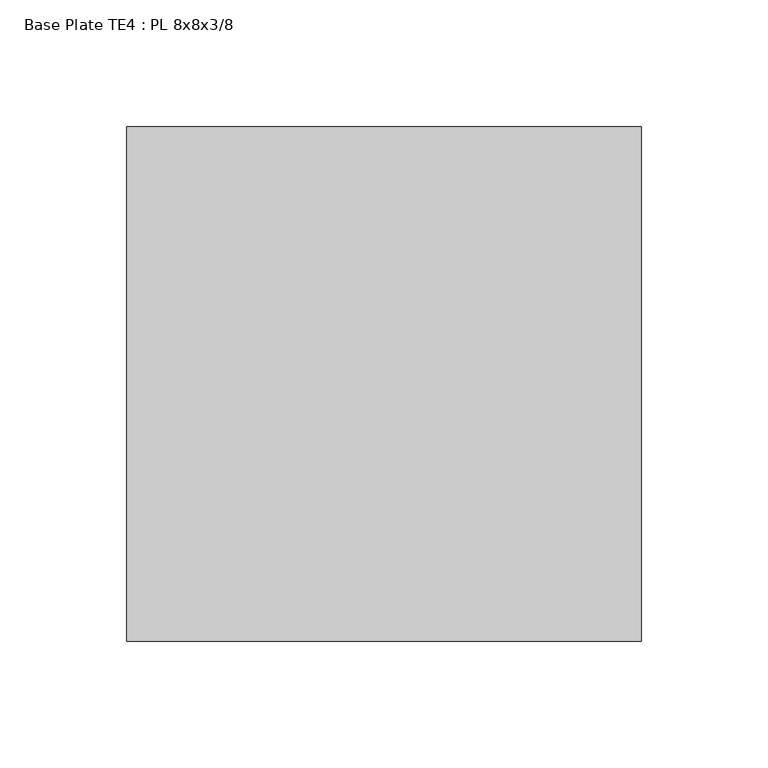
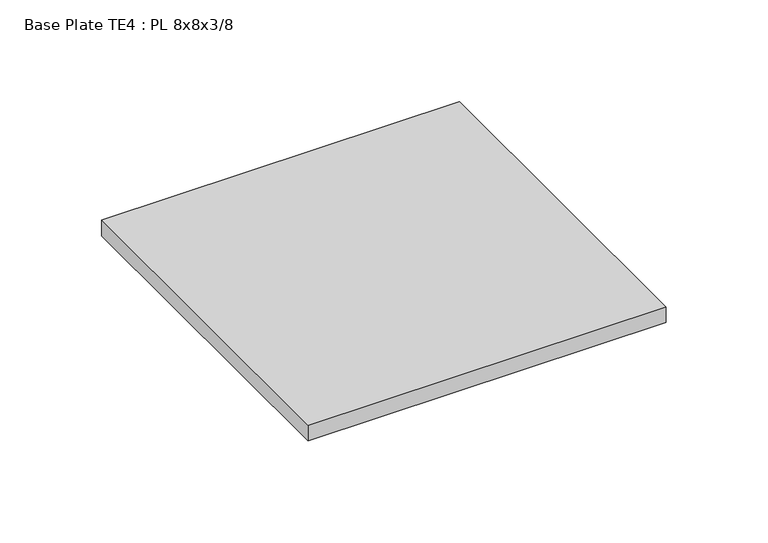
"""IFC4 building model written with IfcOpenShell, lengths in millimetres: proxy geometry, Base Plate TE4 : PL 8x8x3/8."""

from ifc_helpers import new_model, si_unit, frame, origin, place, context, project, spatial, polyline, outline, extrude, source, transform, mapped, element, save


def base_plate_te4_pl_8x8x3_8_c18328d5(model_context):
    return source(origin(), model_context, "Body", "SweptSolid", [
        extrude(outline(polyline([(590318.6599233, -536265.1913841), (590318.6599233, -536468.3913841), (590115.4599233, -536468.3913841), (590115.4599233, -536265.1913841), (590318.6599233, -536265.1913841)])), frame((0.0, 0.0, 19.05), z_axis=(0.0, 0.0, 1.0), x_axis=(1.0, 0.0, 0.0)), (0.0, 0.0, 1.0), 9.525),
    ])


if __name__ == "__main__":
    model = new_model("IFC4")
    model_context = context("Model", 3, world=origin())
    ifc_project = project(units=[si_unit("LENGTHUNIT", "METRE", prefix="MILLI")], contexts=[model_context])
    site = spatial("IfcSite", under=ifc_project)
    building = spatial("IfcBuilding", under=site)
    placement = place(None, origin())
    base_plate_te4_pl_8x8x3_8_shape = base_plate_te4_pl_8x8x3_8_c18328d5(model_context)
    element("IfcBuildingElementProxy", 1, Name="Base Plate TE4 : PL 8x8x3/8", ObjectType="Base Plate TE4 : PL 8x8x3/8", at=placement, inside=building, context=model_context, shape_type="MappedRepresentation", body=[
        mapped(base_plate_te4_pl_8x8x3_8_shape, transform((0.0, 0.0, 0.0), x_axis=(1.0, 0.0, 0.0), y_axis=(0.0, 1.0, 0.0), z_axis=(0.0, 0.0, 1.0))),
    ])
    save(model, "model.ifc")

# Revit data of these elements
# Element 1 (IfcBuildingElementProxy, "Base Plate TE4 : PL 8x8x3/8")
#   Materials on its faces: "GALV. STL BASE PLATE"
# Materials
#   "GALV. STL BASE PLATE": class "Generic", colour RGB 211 211 207, transparency 0, Cost = 0
